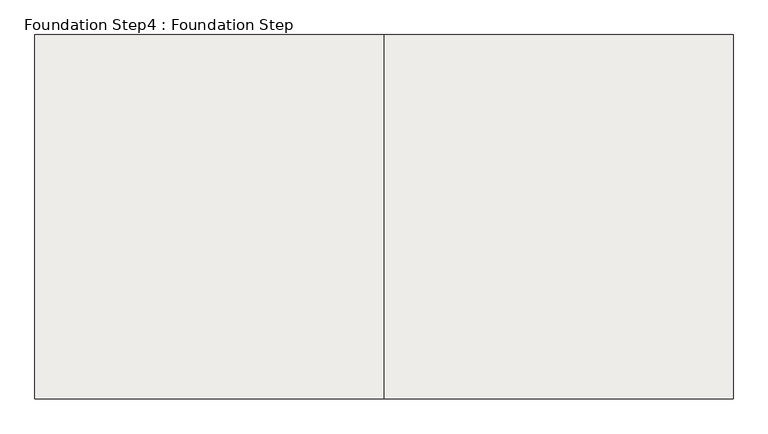
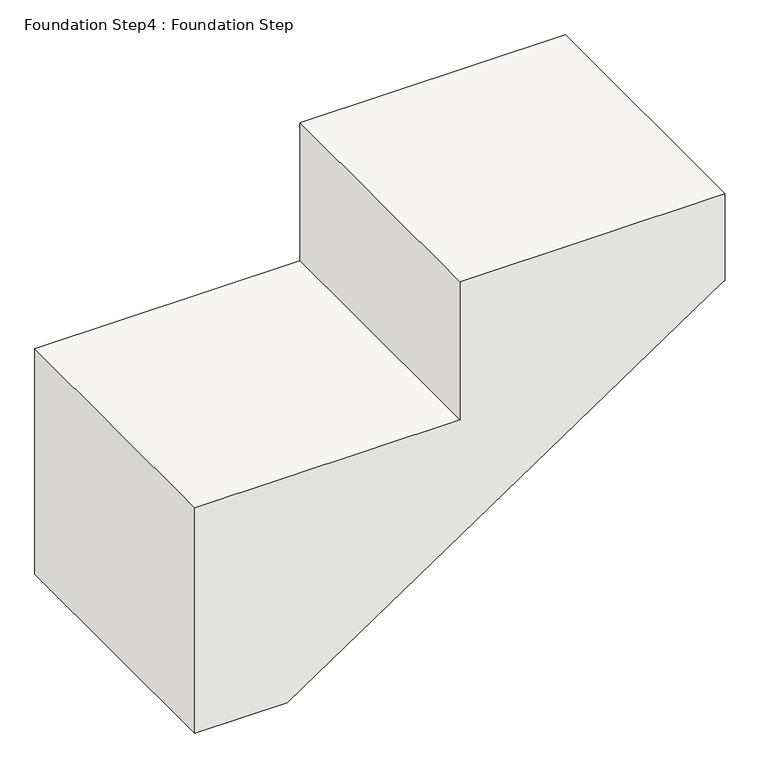
"""IFC4 building model written with IfcOpenShell, lengths in millimetres: slab geometry, Foundation Step4 : Foundation Step."""

import ifcopenshell
import ifcopenshell.guid

model = None  # the IFC model being written
_history = None  # IfcOwnerHistory: only IFC2X3 demands one
_inside = {}  # id of a spatial element -> (the spatial element, [elements in it])
_under = {}  # id of a project, library or spatial element -> (it, [spatial elements below it])
_declared = {}  # id of a project -> (the project, [libraries it declares])
_typed = {}  # id of a type object -> (the type object, [elements of that type])
_made_of = {}  # id of a material, layer set ... -> (it, [elements and type objects made of it])


def new_model(schema):
    """Start an empty IFC model of exactly this schema.

    Asked for "IFC4X3", IfcOpenShell would pick the latest addendum, in which some entities
    have other attributes; the version numbers below select the first issue.
    IFC2X3 requires an IfcOwnerHistory on every rooted entity: one is made here for all.
    """
    global model, _history
    if schema == "IFC4X3":
        model = ifcopenshell.file(schema_version=(4, 3, 0, 0))
    else:
        model = ifcopenshell.file(schema=schema)
    _inside.clear()
    _under.clear()
    _declared.clear()
    _typed.clear()
    _made_of.clear()
    _history = None
    if model.schema == "IFC2X3":
        org = make("IfcOrganization", Name="unknown")
        user = make(
            "IfcPersonAndOrganization",
            ThePerson=make("IfcPerson", FamilyName="unknown"),
            TheOrganization=org,
        )
        app = make(
            "IfcApplication",
            ApplicationDeveloper=org,
            Version="unknown",
            ApplicationFullName="unknown",
            ApplicationIdentifier="unknown",
        )
        _history = make(
            "IfcOwnerHistory",
            OwningUser=user,
            OwningApplication=app,
            ChangeAction="ADDED",
            CreationDate=0,
        )
    return model


def make(cls, **values):
    """One entity of the class cls with the attributes given. An attribute that is None is left unset."""
    return model.create_entity(
        cls, **{name: value for name, value in values.items() if value is not None}
    )


def rooted(cls, **values):
    """An entity with a GlobalId (a new one), such as an element, a storey or a relation."""
    return make(cls, GlobalId=ifcopenshell.guid.new(), OwnerHistory=_history, **values)


def si_unit(unit_type, name, prefix=None):
    """IfcSIUnit, for example si_unit("LENGTHUNIT", "METRE", prefix="MILLI")."""
    return make("IfcSIUnit", UnitType=unit_type, Prefix=prefix, Name=name)


def assignment(units):
    """IfcUnitAssignment: the units of a project."""
    return None if units is None else make("IfcUnitAssignment", Units=units)


def point(xyz):
    """IfcCartesianPoint."""
    return None if xyz is None else make("IfcCartesianPoint", Coordinates=xyz)


def direction(xyz):
    """IfcDirection."""
    return None if xyz is None else make("IfcDirection", DirectionRatios=xyz)


def frame(location, z_axis=None, x_axis=None):
    """IfcAxis2Placement3D, a coordinate frame: its origin and axes. An axis left out is left unset."""
    return make(
        "IfcAxis2Placement3D",
        Location=point(location),
        Axis=direction(z_axis),
        RefDirection=direction(x_axis),
    )


def origin():
    """The frame at (0, 0, 0) with its axes left unset."""
    return frame((0.0, 0.0, 0.0))


def place(relative_to, where):
    """IfcLocalPlacement: puts the frame where relative to a parent placement (None: the world)."""
    return make(
        "IfcLocalPlacement", PlacementRelTo=relative_to, RelativePlacement=where
    )


def context(
    kind, dimensions, precision=None, world=None, true_north=None, identifier=None
):
    """IfcGeometricRepresentationContext, for example the 3D "Model" context."""
    return make(
        "IfcGeometricRepresentationContext",
        ContextIdentifier=identifier,
        ContextType=kind,
        CoordinateSpaceDimension=dimensions,
        Precision=precision,
        WorldCoordinateSystem=world,
        TrueNorth=true_north,
    )


def project(units=None, contexts=None):
    """IfcProject with its units and contexts."""
    return rooted(
        "IfcProject",
        Name="project",
        RepresentationContexts=contexts,
        UnitsInContext=assignment(units),
    )


def spatial(cls, under=None, at=None, **own):
    """A site, building, storey or space (cls), placed at a placement, below another one or the project."""
    s = rooted(cls, ObjectPlacement=at, **own)
    if under is not None:
        _under.setdefault(under.id(), (under, []))[1].append(s)
    return s


def polyline(points):
    """IfcPolyline through the points."""
    return make("IfcPolyline", Points=[point(p) for p in points])


def outline(outer, holes=None, kind="AREA"):
    """IfcArbitraryClosedProfileDef: a profile drawn as a closed curve; with holes, ...WithVoids."""
    if holes is None:
        return make("IfcArbitraryClosedProfileDef", ProfileType=kind, OuterCurve=outer)
    return make(
        "IfcArbitraryProfileDefWithVoids",
        ProfileType=kind,
        OuterCurve=outer,
        InnerCurves=holes,
    )


def extrude(swept, where, along, depth):
    """IfcExtrudedAreaSolid: the profile swept, set in the frame where, extruded along a direction by depth."""
    return make(
        "IfcExtrudedAreaSolid",
        SweptArea=swept,
        Position=where,
        ExtrudedDirection=direction(along),
        Depth=depth,
    )


def shape(context_of_items, identifier, shape_type, items):
    """IfcShapeRepresentation: the items that make up one representation, for example the "Body"."""
    return make(
        "IfcShapeRepresentation",
        ContextOfItems=context_of_items,
        RepresentationIdentifier=identifier,
        RepresentationType=shape_type,
        Items=items,
    )


def source(mapping_origin, context_of_items, identifier, shape_type, items):
    """IfcRepresentationMap: a shape defined once, which mapped items show again and again."""
    return make(
        "IfcRepresentationMap",
        MappingOrigin=mapping_origin,
        MappedRepresentation=shape(context_of_items, identifier, shape_type, items),
    )


def transform(
    local_origin,
    x_axis=None,
    y_axis=None,
    z_axis=None,
    scale=None,
    scale2=None,
    scale3=None,
    uniform=True,
):
    """IfcCartesianTransformationOperator3D, or its non-uniform kind. x_axis, y_axis, z_axis: its Axis1, 2, 3."""
    if uniform:
        return make(
            "IfcCartesianTransformationOperator3D",
            Axis1=direction(x_axis),
            Axis2=direction(y_axis),
            LocalOrigin=point(local_origin),
            Scale=scale,
            Axis3=direction(z_axis),
        )
    return make(
        "IfcCartesianTransformationOperator3DnonUniform",
        Axis1=direction(x_axis),
        Axis2=direction(y_axis),
        LocalOrigin=point(local_origin),
        Scale=scale,
        Axis3=direction(z_axis),
        Scale2=scale2,
        Scale3=scale3,
    )


def mapped(mapping_source, mapping_target):
    """IfcMappedItem: shows the shape of a source again, moved by a transform."""
    return make(
        "IfcMappedItem", MappingSource=mapping_source, MappingTarget=mapping_target
    )


def made_of(thing, what):
    """Note that an element or type object is made of a material, layer set ...; save() writes the relation."""
    if what is not None:
        _made_of.setdefault(what.id(), (what, []))[1].append(thing)
    return thing


def element(
    cls,
    number,
    at=None,
    inside=None,
    cuts=None,
    type_object=None,
    material=None,
    context=None,
    identifier="Body",
    shape_type=None,
    held_by="IfcProductDefinitionShape",
    body=None,
    shapes=None,
    **own,
):
    """One element of the class cls, such as IfcWall. Its Tag is "e" and its number.

    at: its placement. inside: the storey or other place that contains it. cuts: it is an
    opening in that element (IfcRelVoidsElement). A single representation is given by context,
    identifier, shape_type and body (its items); several are given by shapes. held_by: the class
    of the entity that holds the representations. save() writes the other relations.
    """
    e = rooted(cls, Tag="e%d" % number, ObjectPlacement=at, **own)
    if body is not None:
        shapes = [shape(context, identifier, shape_type, body)]
    if shapes is not None:
        e.Representation = make(held_by, Representations=shapes)
    if inside is not None:
        _inside.setdefault(inside.id(), (inside, []))[1].append(e)
    if cuts is not None:
        rooted(
            "IfcRelVoidsElement", RelatingBuildingElement=cuts, RelatedOpeningElement=e
        )
    if type_object is not None:
        _typed.setdefault(type_object.id(), (type_object, []))[1].append(e)
    return made_of(e, material)


def aggregate(whole, parts):
    """IfcRelAggregates: a whole, such as a stair, and the parts it consists of."""
    return rooted("IfcRelAggregates", RelatingObject=whole, RelatedObjects=parts)


def save(model, path):
    """Write the relations noted so far, then the file.

    IfcRelAggregates (storeys below a building ...), IfcRelContainedInSpatialStructure (elements
    in a storey), IfcRelDefinesByType, IfcRelAssociatesMaterial and IfcRelDeclares: one each for
    every whole, place, type object, material and project.
    """
    for whole, parts in _under.values():
        aggregate(whole, parts)
    for where, things in _inside.values():
        rooted(
            "IfcRelContainedInSpatialStructure",
            RelatedElements=things,
            RelatingStructure=where,
        )
    for kind, things in _typed.values():
        rooted("IfcRelDefinesByType", RelatedObjects=things, RelatingType=kind)
    for what, things in _made_of.values():
        rooted("IfcRelAssociatesMaterial", RelatedObjects=things, RelatingMaterial=what)
    for by, libraries in _declared.values():
        rooted("IfcRelDeclares", RelatingContext=by, RelatedDefinitions=libraries)
    model.write(path)


def foundation_step4_foundation_step_7894882b(model_context):
    return source(origin(), model_context, "Body", "SweptSolid", [
        extrude(outline(polyline([(-1092.2, -45178.5909443), (-1574.8, -45178.5909443), (-1574.8, -46054.8909443), (-2362.2, -46054.8909443), (-2362.2, -45750.0909443), (-1397.0, -44308.7600821), (-1397.0, -44302.2909443), (-1092.2, -44302.2909443), (-1092.2, -45178.5909443)])), frame((0.0, -12551.0356529, 0.0), z_axis=(0.0, 1.0, 0.0), x_axis=(0.0, 0.0, 1.0)), (0.0, 0.0, 1.0), 914.4),
    ])


if __name__ == "__main__":
    model = new_model("IFC4")
    model_context = context("Model", 3, world=origin())
    ifc_project = project(units=[si_unit("LENGTHUNIT", "METRE", prefix="MILLI")], contexts=[model_context])
    site = spatial("IfcSite", under=ifc_project)
    building = spatial("IfcBuilding", under=site)
    placement = place(None, origin())
    foundation_step4_foundation_step_shape = foundation_step4_foundation_step_7894882b(model_context)
    element("IfcSlab", 1, ObjectType="Foundation Step4 : Foundation Step", at=placement, inside=building, context=model_context, shape_type="MappedRepresentation", body=[
        mapped(foundation_step4_foundation_step_shape, transform((0.0, 0.0, 0.0), x_axis=(1.0, 0.0, 0.0), y_axis=(0.0, 1.0, 0.0), z_axis=(0.0, 0.0, 1.0))),
    ])
    save(model, "model.ifc")

# Revit data of these elements
# Type "Foundation Step4 : Foundation Step"
#   Structural Material = Concrete, Cast-in-Place gray
# Materials
#   "Concrete, Cast-in-Place gray": class "Concrete", colour RGB 192 192 192, transparency 0, Description = "Cast-in-place concrete", Cost = 0
